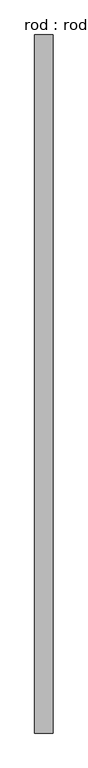
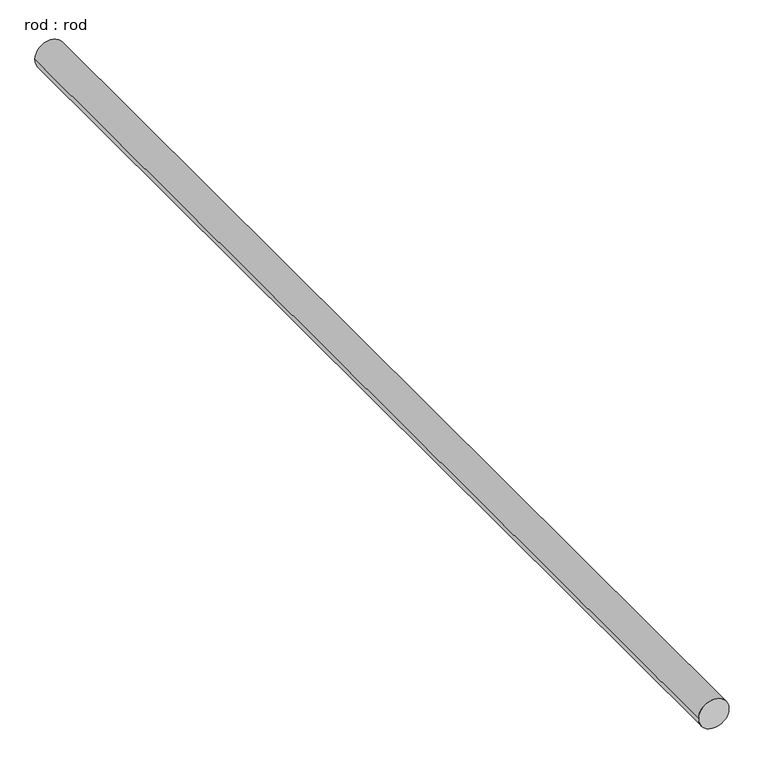
"""IFC4 building model written with IfcOpenShell, lengths in millimetres: proxy geometry, rod : rod."""

from ifc_helpers import new_model, si_unit, point, frame, frame_2d, origin, place, context, project, spatial, circle_curve, trimmed, segment, composite_curve, outline, extrude, source, transform, mapped, element, save


def rod_rod_94f8d9b8(model_context):
    return source(origin(), model_context, "Body", "SweptSolid", [
        extrude(outline(composite_curve([segment(trimmed(circle_curve(frame_2d((0.0108462, 0.0)), 200.0), [point((0.0108462, 200.0))], [point((0.0108462, -200.0))], False, "CARTESIAN"), True, "CONTINUOUS"), segment(trimmed(circle_curve(frame_2d((0.0108462, 0.0)), 200.0), [point((0.0108462, -200.0))], [point((0.0108462, 200.0))], False, "CARTESIAN"), True, "CONTINUOUS")], self_intersect=False)), frame((0.0, -3455.4148857, 0.0), z_axis=(0.0, 1.0, 0.0), x_axis=(0.0, 0.0, 1.0)), (0.0, 0.0, 1.0), 15096.2870021),
    ])


if __name__ == "__main__":
    model = new_model("IFC4")
    model_context = context("Model", 3, world=origin())
    ifc_project = project(units=[si_unit("LENGTHUNIT", "METRE", prefix="MILLI")], contexts=[model_context])
    site = spatial("IfcSite", under=ifc_project)
    building = spatial("IfcBuilding", under=site)
    placement = place(None, origin())
    rod_rod_shape = rod_rod_94f8d9b8(model_context)
    element("IfcBuildingElementProxy", 1, Name="rod : rod", ObjectType="rod : rod", at=placement, inside=building, context=model_context, shape_type="MappedRepresentation", body=[
        mapped(rod_rod_shape, transform((0.0, 0.0, 0.0), x_axis=(1.0, 0.0, 0.0), y_axis=(0.0, 1.0, 0.0), z_axis=(0.0, 0.0, 1.0))),
    ])
    save(model, "model.ifc")

# Revit data of these elements
# Type "rod : rod"
#   Default Elevation = 0
